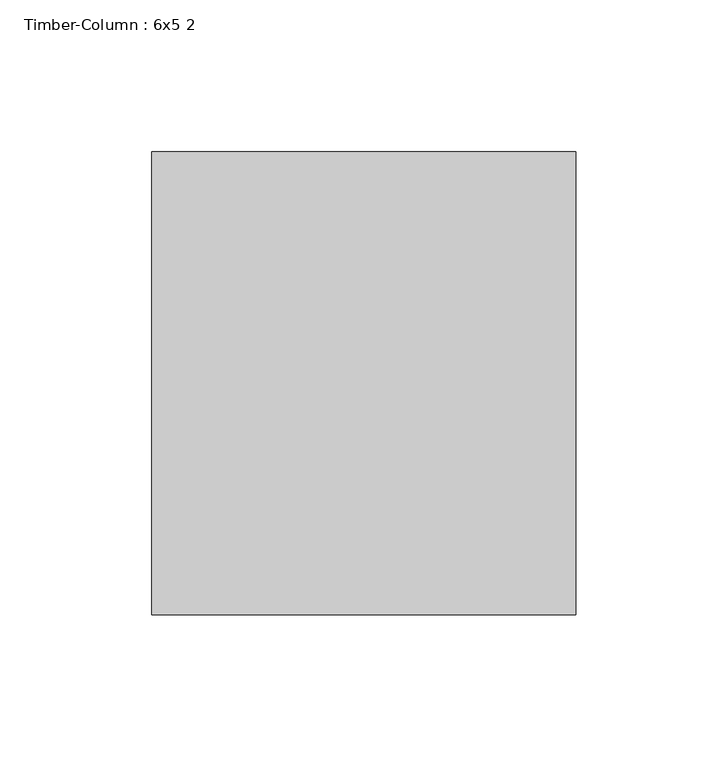
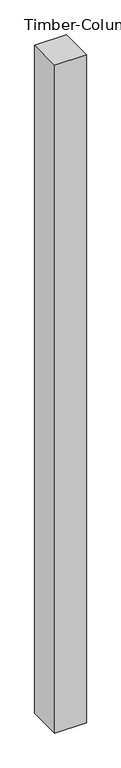
"""IFC4 building model written with IfcOpenShell, lengths in millimetres: column geometry, Timber-Column : 6x5 2."""

import ifcopenshell
import ifcopenshell.guid

model = None  # the IFC model being written
_history = None  # IfcOwnerHistory: only IFC2X3 demands one
_inside = {}  # id of a spatial element -> (the spatial element, [elements in it])
_under = {}  # id of a project, library or spatial element -> (it, [spatial elements below it])
_declared = {}  # id of a project -> (the project, [libraries it declares])
_typed = {}  # id of a type object -> (the type object, [elements of that type])
_made_of = {}  # id of a material, layer set ... -> (it, [elements and type objects made of it])


def new_model(schema):
    """Start an empty IFC model of exactly this schema.

    Asked for "IFC4X3", IfcOpenShell would pick the latest addendum, in which some entities
    have other attributes; the version numbers below select the first issue.
    IFC2X3 requires an IfcOwnerHistory on every rooted entity: one is made here for all.
    """
    global model, _history
    if schema == "IFC4X3":
        model = ifcopenshell.file(schema_version=(4, 3, 0, 0))
    else:
        model = ifcopenshell.file(schema=schema)
    _inside.clear()
    _under.clear()
    _declared.clear()
    _typed.clear()
    _made_of.clear()
    _history = None
    if model.schema == "IFC2X3":
        org = make("IfcOrganization", Name="unknown")
        user = make(
            "IfcPersonAndOrganization",
            ThePerson=make("IfcPerson", FamilyName="unknown"),
            TheOrganization=org,
        )
        app = make(
            "IfcApplication",
            ApplicationDeveloper=org,
            Version="unknown",
            ApplicationFullName="unknown",
            ApplicationIdentifier="unknown",
        )
        _history = make(
            "IfcOwnerHistory",
            OwningUser=user,
            OwningApplication=app,
            ChangeAction="ADDED",
            CreationDate=0,
        )
    return model


def make(cls, **values):
    """One entity of the class cls with the attributes given. An attribute that is None is left unset."""
    return model.create_entity(
        cls, **{name: value for name, value in values.items() if value is not None}
    )


def rooted(cls, **values):
    """An entity with a GlobalId (a new one), such as an element, a storey or a relation."""
    return make(cls, GlobalId=ifcopenshell.guid.new(), OwnerHistory=_history, **values)


def si_unit(unit_type, name, prefix=None):
    """IfcSIUnit, for example si_unit("LENGTHUNIT", "METRE", prefix="MILLI")."""
    return make("IfcSIUnit", UnitType=unit_type, Prefix=prefix, Name=name)


def assignment(units):
    """IfcUnitAssignment: the units of a project."""
    return None if units is None else make("IfcUnitAssignment", Units=units)


def point(xyz):
    """IfcCartesianPoint."""
    return None if xyz is None else make("IfcCartesianPoint", Coordinates=xyz)


def direction(xyz):
    """IfcDirection."""
    return None if xyz is None else make("IfcDirection", DirectionRatios=xyz)


def frame(location, z_axis=None, x_axis=None):
    """IfcAxis2Placement3D, a coordinate frame: its origin and axes. An axis left out is left unset."""
    return make(
        "IfcAxis2Placement3D",
        Location=point(location),
        Axis=direction(z_axis),
        RefDirection=direction(x_axis),
    )


def origin():
    """The frame at (0, 0, 0) with its axes left unset."""
    return frame((0.0, 0.0, 0.0))


def origin_with_axes():
    """The frame at (0, 0, 0) with the z axis (0, 0, 1) and the x axis (1, 0, 0) written out."""
    return frame((0.0, 0.0, 0.0), z_axis=(0.0, 0.0, 1.0), x_axis=(1.0, 0.0, 0.0))


def place(relative_to, where):
    """IfcLocalPlacement: puts the frame where relative to a parent placement (None: the world)."""
    return make(
        "IfcLocalPlacement", PlacementRelTo=relative_to, RelativePlacement=where
    )


def context(
    kind, dimensions, precision=None, world=None, true_north=None, identifier=None
):
    """IfcGeometricRepresentationContext, for example the 3D "Model" context."""
    return make(
        "IfcGeometricRepresentationContext",
        ContextIdentifier=identifier,
        ContextType=kind,
        CoordinateSpaceDimension=dimensions,
        Precision=precision,
        WorldCoordinateSystem=world,
        TrueNorth=true_north,
    )


def project(units=None, contexts=None):
    """IfcProject with its units and contexts."""
    return rooted(
        "IfcProject",
        Name="project",
        RepresentationContexts=contexts,
        UnitsInContext=assignment(units),
    )


def spatial(cls, under=None, at=None, **own):
    """A site, building, storey or space (cls), placed at a placement, below another one or the project."""
    s = rooted(cls, ObjectPlacement=at, **own)
    if under is not None:
        _under.setdefault(under.id(), (under, []))[1].append(s)
    return s


def polyline(points):
    """IfcPolyline through the points."""
    return make("IfcPolyline", Points=[point(p) for p in points])


def outline(outer, holes=None, kind="AREA"):
    """IfcArbitraryClosedProfileDef: a profile drawn as a closed curve; with holes, ...WithVoids."""
    if holes is None:
        return make("IfcArbitraryClosedProfileDef", ProfileType=kind, OuterCurve=outer)
    return make(
        "IfcArbitraryProfileDefWithVoids",
        ProfileType=kind,
        OuterCurve=outer,
        InnerCurves=holes,
    )


def extrude(swept, where, along, depth):
    """IfcExtrudedAreaSolid: the profile swept, set in the frame where, extruded along a direction by depth."""
    return make(
        "IfcExtrudedAreaSolid",
        SweptArea=swept,
        Position=where,
        ExtrudedDirection=direction(along),
        Depth=depth,
    )


def shape(context_of_items, identifier, shape_type, items):
    """IfcShapeRepresentation: the items that make up one representation, for example the "Body"."""
    return make(
        "IfcShapeRepresentation",
        ContextOfItems=context_of_items,
        RepresentationIdentifier=identifier,
        RepresentationType=shape_type,
        Items=items,
    )


def source(mapping_origin, context_of_items, identifier, shape_type, items):
    """IfcRepresentationMap: a shape defined once, which mapped items show again and again."""
    return make(
        "IfcRepresentationMap",
        MappingOrigin=mapping_origin,
        MappedRepresentation=shape(context_of_items, identifier, shape_type, items),
    )


def transform(
    local_origin,
    x_axis=None,
    y_axis=None,
    z_axis=None,
    scale=None,
    scale2=None,
    scale3=None,
    uniform=True,
):
    """IfcCartesianTransformationOperator3D, or its non-uniform kind. x_axis, y_axis, z_axis: its Axis1, 2, 3."""
    if uniform:
        return make(
            "IfcCartesianTransformationOperator3D",
            Axis1=direction(x_axis),
            Axis2=direction(y_axis),
            LocalOrigin=point(local_origin),
            Scale=scale,
            Axis3=direction(z_axis),
        )
    return make(
        "IfcCartesianTransformationOperator3DnonUniform",
        Axis1=direction(x_axis),
        Axis2=direction(y_axis),
        LocalOrigin=point(local_origin),
        Scale=scale,
        Axis3=direction(z_axis),
        Scale2=scale2,
        Scale3=scale3,
    )


def mapped(mapping_source, mapping_target):
    """IfcMappedItem: shows the shape of a source again, moved by a transform."""
    return make(
        "IfcMappedItem", MappingSource=mapping_source, MappingTarget=mapping_target
    )


def made_of(thing, what):
    """Note that an element or type object is made of a material, layer set ...; save() writes the relation."""
    if what is not None:
        _made_of.setdefault(what.id(), (what, []))[1].append(thing)
    return thing


def element(
    cls,
    number,
    at=None,
    inside=None,
    cuts=None,
    type_object=None,
    material=None,
    context=None,
    identifier="Body",
    shape_type=None,
    held_by="IfcProductDefinitionShape",
    body=None,
    shapes=None,
    **own,
):
    """One element of the class cls, such as IfcWall. Its Tag is "e" and its number.

    at: its placement. inside: the storey or other place that contains it. cuts: it is an
    opening in that element (IfcRelVoidsElement). A single representation is given by context,
    identifier, shape_type and body (its items); several are given by shapes. held_by: the class
    of the entity that holds the representations. save() writes the other relations.
    """
    e = rooted(cls, Tag="e%d" % number, ObjectPlacement=at, **own)
    if body is not None:
        shapes = [shape(context, identifier, shape_type, body)]
    if shapes is not None:
        e.Representation = make(held_by, Representations=shapes)
    if inside is not None:
        _inside.setdefault(inside.id(), (inside, []))[1].append(e)
    if cuts is not None:
        rooted(
            "IfcRelVoidsElement", RelatingBuildingElement=cuts, RelatedOpeningElement=e
        )
    if type_object is not None:
        _typed.setdefault(type_object.id(), (type_object, []))[1].append(e)
    return made_of(e, material)


def aggregate(whole, parts):
    """IfcRelAggregates: a whole, such as a stair, and the parts it consists of."""
    return rooted("IfcRelAggregates", RelatingObject=whole, RelatedObjects=parts)


def save(model, path):
    """Write the relations noted so far, then the file.

    IfcRelAggregates (storeys below a building ...), IfcRelContainedInSpatialStructure (elements
    in a storey), IfcRelDefinesByType, IfcRelAssociatesMaterial and IfcRelDeclares: one each for
    every whole, place, type object, material and project.
    """
    for whole, parts in _under.values():
        aggregate(whole, parts)
    for where, things in _inside.values():
        rooted(
            "IfcRelContainedInSpatialStructure",
            RelatedElements=things,
            RelatingStructure=where,
        )
    for kind, things in _typed.values():
        rooted("IfcRelDefinesByType", RelatedObjects=things, RelatingType=kind)
    for what, things in _made_of.values():
        rooted("IfcRelAssociatesMaterial", RelatedObjects=things, RelatingMaterial=what)
    for by, libraries in _declared.values():
        rooted("IfcRelDeclares", RelatingContext=by, RelatedDefinitions=libraries)
    model.write(path)


def timber_column_6x5_2_9af8efbf(model_context):
    return source(origin(), model_context, "Body", "SweptSolid", [
        extrude(outline(polyline([(69.85, 76.2), (69.85, -76.2), (-69.85, -76.2), (-69.85, 76.2), (69.85, 76.2)])), origin_with_axes(), (0.0, 0.0, 1.0), 3111.5),
    ])


if __name__ == "__main__":
    model = new_model("IFC4")
    model_context = context("Model", 3, world=origin())
    ifc_project = project(units=[si_unit("LENGTHUNIT", "METRE", prefix="MILLI")], contexts=[model_context])
    site = spatial("IfcSite", under=ifc_project)
    building = spatial("IfcBuilding", under=site)
    placement = place(None, origin())
    timber_column_6x5_2_shape = timber_column_6x5_2_9af8efbf(model_context)
    element("IfcColumn", 1, ObjectType="Timber-Column : 6x5 2", at=placement, inside=building, context=model_context, shape_type="MappedRepresentation", body=[
        mapped(timber_column_6x5_2_shape, transform((0.0, 0.0, 0.0), x_axis=(1.0, 0.0, 0.0), y_axis=(0.0, 1.0, 0.0), z_axis=(0.0, 0.0, 1.0))),
    ])
    save(model, "model.ifc")

# Revit data of these elements
# Type "Timber-Column : 6x5 2"
#   Assembly Code = "B10"
#   A = 0.140625 SF
#   b = 0' - 5 1/2"
#   d = 0' - 6"
#   Structural Material [instance default] = Softwood, Lumber
# Element 1 (IfcColumn, "Timber-Column : 6x5 2")
#   Materials on its faces: "Softwood, Lumber"
# Materials
#   "Softwood, Lumber": class "Wood", colour RGB 144 113 62, transparency 0, Description = "Pinus Echinata", Cost = 0
